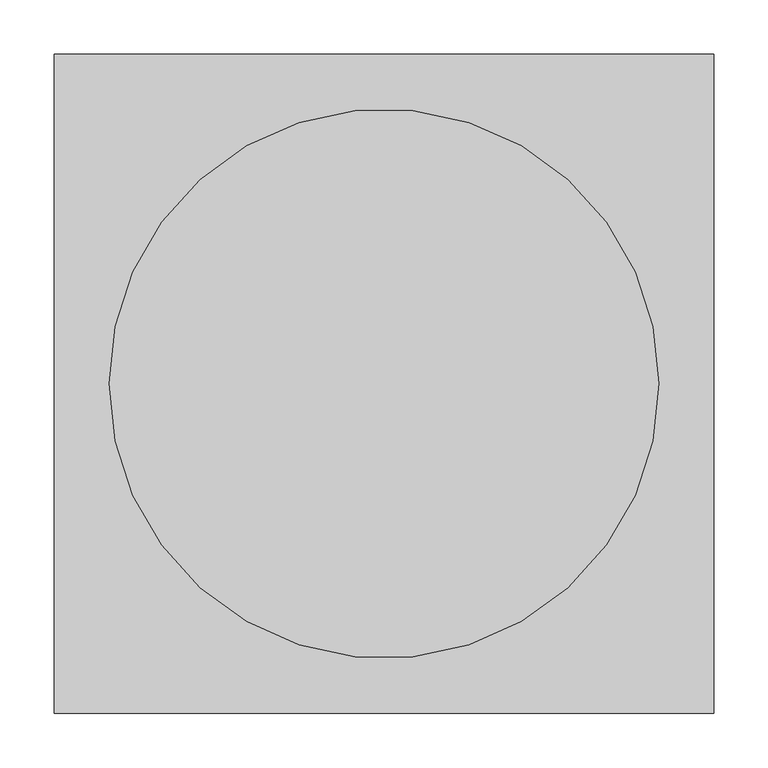
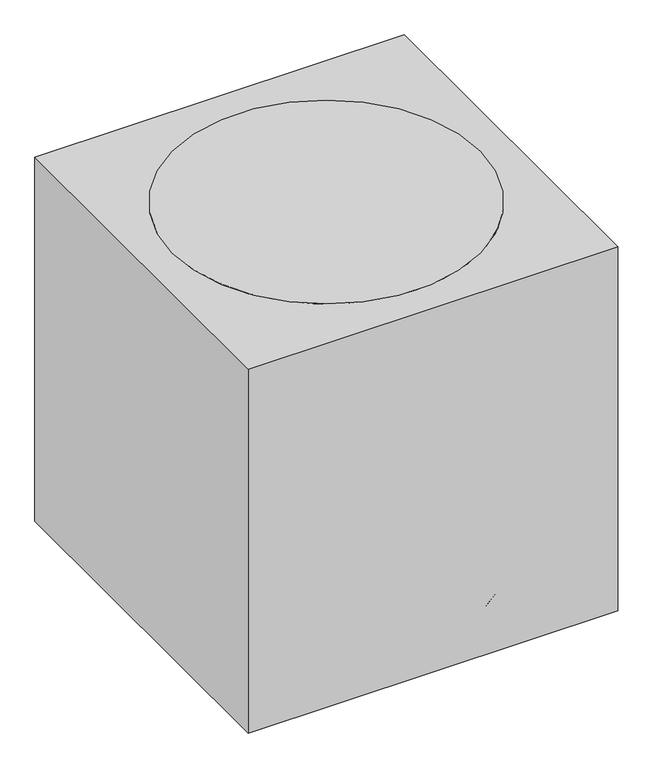
"""IFC4 building model written with IfcOpenShell, lengths in millimetres: proxy geometry, M5030 - Stool, Surgeon, Revolving : M5030 - Stool, Surgeon, Revolving."""

import ifcopenshell
import ifcopenshell.guid

model = None  # the IFC model being written
_history = None  # IfcOwnerHistory: only IFC2X3 demands one
_inside = {}  # id of a spatial element -> (the spatial element, [elements in it])
_under = {}  # id of a project, library or spatial element -> (it, [spatial elements below it])
_declared = {}  # id of a project -> (the project, [libraries it declares])
_typed = {}  # id of a type object -> (the type object, [elements of that type])
_made_of = {}  # id of a material, layer set ... -> (it, [elements and type objects made of it])


def new_model(schema):
    """Start an empty IFC model of exactly this schema.

    Asked for "IFC4X3", IfcOpenShell would pick the latest addendum, in which some entities
    have other attributes; the version numbers below select the first issue.
    IFC2X3 requires an IfcOwnerHistory on every rooted entity: one is made here for all.
    """
    global model, _history
    if schema == "IFC4X3":
        model = ifcopenshell.file(schema_version=(4, 3, 0, 0))
    else:
        model = ifcopenshell.file(schema=schema)
    _inside.clear()
    _under.clear()
    _declared.clear()
    _typed.clear()
    _made_of.clear()
    _history = None
    if model.schema == "IFC2X3":
        org = make("IfcOrganization", Name="unknown")
        user = make(
            "IfcPersonAndOrganization",
            ThePerson=make("IfcPerson", FamilyName="unknown"),
            TheOrganization=org,
        )
        app = make(
            "IfcApplication",
            ApplicationDeveloper=org,
            Version="unknown",
            ApplicationFullName="unknown",
            ApplicationIdentifier="unknown",
        )
        _history = make(
            "IfcOwnerHistory",
            OwningUser=user,
            OwningApplication=app,
            ChangeAction="ADDED",
            CreationDate=0,
        )
    return model


def make(cls, **values):
    """One entity of the class cls with the attributes given. An attribute that is None is left unset."""
    return model.create_entity(
        cls, **{name: value for name, value in values.items() if value is not None}
    )


def rooted(cls, **values):
    """An entity with a GlobalId (a new one), such as an element, a storey or a relation."""
    return make(cls, GlobalId=ifcopenshell.guid.new(), OwnerHistory=_history, **values)


def si_unit(unit_type, name, prefix=None):
    """IfcSIUnit, for example si_unit("LENGTHUNIT", "METRE", prefix="MILLI")."""
    return make("IfcSIUnit", UnitType=unit_type, Prefix=prefix, Name=name)


def assignment(units):
    """IfcUnitAssignment: the units of a project."""
    return None if units is None else make("IfcUnitAssignment", Units=units)


def point(xyz):
    """IfcCartesianPoint."""
    return None if xyz is None else make("IfcCartesianPoint", Coordinates=xyz)


def direction(xyz):
    """IfcDirection."""
    return None if xyz is None else make("IfcDirection", DirectionRatios=xyz)


def frame(location, z_axis=None, x_axis=None):
    """IfcAxis2Placement3D, a coordinate frame: its origin and axes. An axis left out is left unset."""
    return make(
        "IfcAxis2Placement3D",
        Location=point(location),
        Axis=direction(z_axis),
        RefDirection=direction(x_axis),
    )


def frame_2d(location, x_axis=None):
    """IfcAxis2Placement2D, a coordinate frame in the plane: its origin and x axis."""
    return make(
        "IfcAxis2Placement2D", Location=point(location), RefDirection=direction(x_axis)
    )


def origin():
    """The frame at (0, 0, 0) with its axes left unset."""
    return frame((0.0, 0.0, 0.0))


def origin_with_axes():
    """The frame at (0, 0, 0) with the z axis (0, 0, 1) and the x axis (1, 0, 0) written out."""
    return frame((0.0, 0.0, 0.0), z_axis=(0.0, 0.0, 1.0), x_axis=(1.0, 0.0, 0.0))


def origin_2d():
    """The frame at (0, 0) in the plane with its x axis left unset."""
    return frame_2d((0.0, 0.0))


def place(relative_to, where):
    """IfcLocalPlacement: puts the frame where relative to a parent placement (None: the world)."""
    return make(
        "IfcLocalPlacement", PlacementRelTo=relative_to, RelativePlacement=where
    )


def context(
    kind, dimensions, precision=None, world=None, true_north=None, identifier=None
):
    """IfcGeometricRepresentationContext, for example the 3D "Model" context."""
    return make(
        "IfcGeometricRepresentationContext",
        ContextIdentifier=identifier,
        ContextType=kind,
        CoordinateSpaceDimension=dimensions,
        Precision=precision,
        WorldCoordinateSystem=world,
        TrueNorth=true_north,
    )


def project(units=None, contexts=None):
    """IfcProject with its units and contexts."""
    return rooted(
        "IfcProject",
        Name="project",
        RepresentationContexts=contexts,
        UnitsInContext=assignment(units),
    )


def spatial(cls, under=None, at=None, **own):
    """A site, building, storey or space (cls), placed at a placement, below another one or the project."""
    s = rooted(cls, ObjectPlacement=at, **own)
    if under is not None:
        _under.setdefault(under.id(), (under, []))[1].append(s)
    return s


def polyline(points):
    """IfcPolyline through the points."""
    return make("IfcPolyline", Points=[point(p) for p in points])


def circle_curve(where, radius):
    """IfcCircle in the frame where."""
    return make("IfcCircle", Position=where, Radius=radius)


def trimmed(basis, trim1, trim2, sense, master):
    """IfcTrimmedCurve: the piece of a basis curve between two trims."""
    return make(
        "IfcTrimmedCurve",
        BasisCurve=basis,
        Trim1=trim1,
        Trim2=trim2,
        SenseAgreement=sense,
        MasterRepresentation=master,
    )


def segment(curve, same_sense, transition):
    """IfcCompositeCurveSegment."""
    return make(
        "IfcCompositeCurveSegment",
        Transition=transition,
        SameSense=same_sense,
        ParentCurve=curve,
    )


def composite_curve(segments, self_intersect=None):
    """IfcCompositeCurve: segments joined end to end."""
    return make("IfcCompositeCurve", Segments=segments, SelfIntersect=self_intersect)


def outline(outer, holes=None, kind="AREA"):
    """IfcArbitraryClosedProfileDef: a profile drawn as a closed curve; with holes, ...WithVoids."""
    if holes is None:
        return make("IfcArbitraryClosedProfileDef", ProfileType=kind, OuterCurve=outer)
    return make(
        "IfcArbitraryProfileDefWithVoids",
        ProfileType=kind,
        OuterCurve=outer,
        InnerCurves=holes,
    )


def extrude(swept, where, along, depth):
    """IfcExtrudedAreaSolid: the profile swept, set in the frame where, extruded along a direction by depth."""
    return make(
        "IfcExtrudedAreaSolid",
        SweptArea=swept,
        Position=where,
        ExtrudedDirection=direction(along),
        Depth=depth,
    )


def shape(context_of_items, identifier, shape_type, items):
    """IfcShapeRepresentation: the items that make up one representation, for example the "Body"."""
    return make(
        "IfcShapeRepresentation",
        ContextOfItems=context_of_items,
        RepresentationIdentifier=identifier,
        RepresentationType=shape_type,
        Items=items,
    )


def source(mapping_origin, context_of_items, identifier, shape_type, items):
    """IfcRepresentationMap: a shape defined once, which mapped items show again and again."""
    return make(
        "IfcRepresentationMap",
        MappingOrigin=mapping_origin,
        MappedRepresentation=shape(context_of_items, identifier, shape_type, items),
    )


def transform(
    local_origin,
    x_axis=None,
    y_axis=None,
    z_axis=None,
    scale=None,
    scale2=None,
    scale3=None,
    uniform=True,
):
    """IfcCartesianTransformationOperator3D, or its non-uniform kind. x_axis, y_axis, z_axis: its Axis1, 2, 3."""
    if uniform:
        return make(
            "IfcCartesianTransformationOperator3D",
            Axis1=direction(x_axis),
            Axis2=direction(y_axis),
            LocalOrigin=point(local_origin),
            Scale=scale,
            Axis3=direction(z_axis),
        )
    return make(
        "IfcCartesianTransformationOperator3DnonUniform",
        Axis1=direction(x_axis),
        Axis2=direction(y_axis),
        LocalOrigin=point(local_origin),
        Scale=scale,
        Axis3=direction(z_axis),
        Scale2=scale2,
        Scale3=scale3,
    )


def mapped(mapping_source, mapping_target):
    """IfcMappedItem: shows the shape of a source again, moved by a transform."""
    return make(
        "IfcMappedItem", MappingSource=mapping_source, MappingTarget=mapping_target
    )


def made_of(thing, what):
    """Note that an element or type object is made of a material, layer set ...; save() writes the relation."""
    if what is not None:
        _made_of.setdefault(what.id(), (what, []))[1].append(thing)
    return thing


def element(
    cls,
    number,
    at=None,
    inside=None,
    cuts=None,
    type_object=None,
    material=None,
    context=None,
    identifier="Body",
    shape_type=None,
    held_by="IfcProductDefinitionShape",
    body=None,
    shapes=None,
    **own,
):
    """One element of the class cls, such as IfcWall. Its Tag is "e" and its number.

    at: its placement. inside: the storey or other place that contains it. cuts: it is an
    opening in that element (IfcRelVoidsElement). A single representation is given by context,
    identifier, shape_type and body (its items); several are given by shapes. held_by: the class
    of the entity that holds the representations. save() writes the other relations.
    """
    e = rooted(cls, Tag="e%d" % number, ObjectPlacement=at, **own)
    if body is not None:
        shapes = [shape(context, identifier, shape_type, body)]
    if shapes is not None:
        e.Representation = make(held_by, Representations=shapes)
    if inside is not None:
        _inside.setdefault(inside.id(), (inside, []))[1].append(e)
    if cuts is not None:
        rooted(
            "IfcRelVoidsElement", RelatingBuildingElement=cuts, RelatedOpeningElement=e
        )
    if type_object is not None:
        _typed.setdefault(type_object.id(), (type_object, []))[1].append(e)
    return made_of(e, material)


def aggregate(whole, parts):
    """IfcRelAggregates: a whole, such as a stair, and the parts it consists of."""
    return rooted("IfcRelAggregates", RelatingObject=whole, RelatedObjects=parts)


def save(model, path):
    """Write the relations noted so far, then the file.

    IfcRelAggregates (storeys below a building ...), IfcRelContainedInSpatialStructure (elements
    in a storey), IfcRelDefinesByType, IfcRelAssociatesMaterial and IfcRelDeclares: one each for
    every whole, place, type object, material and project.
    """
    for whole, parts in _under.values():
        aggregate(whole, parts)
    for where, things in _inside.values():
        rooted(
            "IfcRelContainedInSpatialStructure",
            RelatedElements=things,
            RelatingStructure=where,
        )
    for kind, things in _typed.values():
        rooted("IfcRelDefinesByType", RelatedObjects=things, RelatingType=kind)
    for what, things in _made_of.values():
        rooted("IfcRelAssociatesMaterial", RelatedObjects=things, RelatingMaterial=what)
    for by, libraries in _declared.values():
        rooted("IfcRelDeclares", RelatingContext=by, RelatedDefinitions=libraries)
    model.write(path)


def specialty_equipment_4e63f546(model_context):
    return source(origin(), model_context, "Body", "SweptSolid", [
        extrude(outline(composite_curve([segment(trimmed(circle_curve(origin_2d(), 254.0), [point((-254.0, 0.0))], [point((254.0, 0.0))], False, "CARTESIAN"), True, "CONTINUOUS"), segment(trimmed(circle_curve(origin_2d(), 254.0), [point((254.0, 0.0))], [point((-254.0, 0.0))], False, "CARTESIAN"), True, "CONTINUOUS")], self_intersect=False)), frame((0.0, 0.0, 584.2), z_axis=(0.0, 0.0, 1.0), x_axis=(1.0, 0.0, 0.0)), (0.0, 0.0, 1.0), 50.8),
        extrude(outline(composite_curve([segment(trimmed(circle_curve(frame_2d((0.0, -25.7612183)), 25.7612183), [point((0.0, -51.5224365))], [point((0.0, 0.0))], False, "CARTESIAN"), True, "CONTINUOUS"), segment(trimmed(circle_curve(frame_2d((0.0, -25.7612183)), 25.7612183), [point((0.0, 0.0))], [point((0.0, -51.5224365))], False, "CARTESIAN"), True, "CONTINUOUS")], self_intersect=False)), frame((203.8559823, 49.544861, 25.7612183), z_axis=(-0.3090169943748919, 0.9510565162951716, 0.0), x_axis=(0.0, 0.0, -1.0)), (0.0, 0.0, 1.0), 31.75),
        extrude(outline(composite_curve([segment(polyline([(-57.1058784, 0.0), (-0.678315, 0.0)]), True, "CONTINUOUS"), segment(trimmed(circle_curve(frame_2d((-28.8920968, 0.0)), 28.2137817), [point((-0.678315, 0.0))], [point((-57.1058784, 0.0))], False, "CARTESIAN"), True, "CONTINUOUS")], self_intersect=False)), frame((256.8155026, 63.4140597, 25.7612183), z_axis=(-0.30901699437489183, 0.9510565162951716, 0.0), x_axis=(0.9510565162951716, 0.30901699437489183, 0.0)), (0.0, 0.0, 1.0), 38.1),
        extrude(outline(composite_curve([segment(trimmed(circle_curve(frame_2d((223.4509477, 72.6028121)), 3.5091751), [point((222.3665529, 75.940236))], [point((224.5353424, 69.2653883))], False, "CARTESIAN"), True, "CONTINUOUS"), segment(trimmed(circle_curve(frame_2d((223.4509477, 72.6028121)), 3.5091751), [point((224.5353424, 69.2653883))], [point((222.3665529, 75.940236))], False, "CARTESIAN"), True, "CONTINUOUS")], self_intersect=False)), frame((0.0, 0.0, 53.975), z_axis=(0.0, 0.0, 1.0), x_axis=(1.0, 0.0, 0.0)), (0.0, 0.0, 1.0), 13.49375),
        extrude(outline(polyline([(230.0293313, 68.0638809), (25.3978935, 1.5750963), (21.4736172, 13.6527769), (226.105055, 80.1415615), (230.0293313, 68.0638809)])), frame((0.0, 0.0, 67.46875), z_axis=(0.0, 0.0, 1.0), x_axis=(1.0, 0.0, 0.0)), (0.0, 0.0, 1.0), 50.8),
        extrude(outline(composite_curve([segment(trimmed(circle_curve(frame_2d((0.0, -25.7612182)), 25.7612183), [point((0.0, -51.5224365))], [point((0.0, 0.0))], False, "CARTESIAN"), True, "CONTINUOUS"), segment(trimmed(circle_curve(frame_2d((0.0, -25.7612182)), 25.7612183), [point((0.0, 0.0))], [point((0.0, -51.5224365))], False, "CARTESIAN"), True, "CONTINUOUS")], self_intersect=False)), frame((110.1149259, -178.5683563, 25.7612183), z_axis=(0.8090169943749846, 0.5877852522924221, 0.0), x_axis=(0.0, 0.0, -1.0)), (0.0, 0.0, 1.0), 31.75),
        extrude(outline(composite_curve([segment(polyline([(-57.1058785, 0.0), (-0.6783149, 0.0)]), True, "CONTINUOUS"), segment(trimmed(circle_curve(frame_2d((-28.8920966, 0.0)), 28.2137817), [point((-0.6783149, 0.0))], [point((-57.1058785, 0.0))], False, "CARTESIAN"), True, "CONTINUOUS")], self_intersect=False)), frame((139.6707094, -224.6500351, 25.7612183), z_axis=(0.8090169943749845, 0.5877852522924222, 0.0), x_axis=(0.5877852522924222, -0.8090169943749845, 0.0)), (0.0, 0.0, 1.0), 38.1),
        extrude(outline(composite_curve([segment(trimmed(circle_curve(frame_2d((138.0995178, -190.0789771)), 3.5091751), [point((140.9385001, -188.0163357))], [point((135.2605355, -192.1416185))], False, "CARTESIAN"), True, "CONTINUOUS"), segment(trimmed(circle_curve(frame_2d((138.0995178, -190.0789771)), 3.5091751), [point((135.2605355, -192.1416185))], [point((140.9385001, -188.0163357))], False, "CARTESIAN"), True, "CONTINUOUS")], self_intersect=False)), frame((0.0, 0.0, 53.975), z_axis=(0.0, 0.0, 1.0), x_axis=(1.0, 0.0, 0.0)), (0.0, 0.0, 1.0), 13.49375),
        extrude(outline(polyline([(135.81557, -197.7379985), (9.3463863, -23.6681006), (19.620275, -16.2036835), (146.0894588, -190.2735815), (135.81557, -197.7379985)])), frame((0.0, 0.0, 67.46875), z_axis=(0.0, 0.0, 1.0), x_axis=(1.0, 0.0, 0.0)), (0.0, 0.0, 1.0), 50.8),
        extrude(outline(composite_curve([segment(trimmed(circle_curve(frame_2d((0.0, -25.7612182)), 25.7612183), [point((0.0, -51.5224365))], [point((0.0, 0.0))], False, "CARTESIAN"), True, "CONTINUOUS"), segment(trimmed(circle_curve(frame_2d((0.0, -25.7612182)), 25.7612183), [point((0.0, 0.0))], [point((0.0, -51.5224365))], False, "CARTESIAN"), True, "CONTINUOUS")], self_intersect=False)), frame((-110.1149259, -178.5683563, 25.7612183), z_axis=(-0.8090169943749151, 0.5877852522925178, 0.0), x_axis=(0.0, 0.0, 1.0)), (0.0, 0.0, 1.0), 31.75),
        extrude(outline(composite_curve([segment(trimmed(circle_curve(frame_2d((28.8920966, 0.0)), 28.2137817), [point((57.1058785, 0.0))], [point((0.6783149, 0.0))], False, "CARTESIAN"), True, "CONTINUOUS"), segment(polyline([(0.6783149, 0.0), (57.1058785, 0.0)]), True, "CONTINUOUS")], self_intersect=False)), frame((-139.6707094, -224.6500351, 25.7612183), z_axis=(-0.809016994374915, 0.5877852522925177, 0.0), x_axis=(0.5877852522925177, 0.809016994374915, 0.0)), (0.0, 0.0, 1.0), 38.1),
        extrude(outline(composite_curve([segment(trimmed(circle_curve(frame_2d((-138.1007518, -190.0780805)), 3.5091751), [point((-135.2617695, -192.1407219))], [point((-140.9397341, -188.0154391))], False, "CARTESIAN"), True, "CONTINUOUS"), segment(trimmed(circle_curve(frame_2d((-138.1007518, -190.0780805)), 3.5091751), [point((-140.9397341, -188.0154391))], [point((-135.2617695, -192.1407219))], False, "CARTESIAN"), True, "CONTINUOUS")], self_intersect=False)), frame((0.0, 0.0, 53.975), z_axis=(0.0, 0.0, 1.0), x_axis=(1.0, 0.0, 0.0)), (0.0, 0.0, 1.0), 13.49375),
        extrude(outline(polyline([(-146.0906928, -190.2726849), (-19.6215091, -16.2027869), (-9.3476203, -23.667204), (-135.8168041, -197.737102), (-146.0906928, -190.2726849)])), frame((0.0, 0.0, 67.46875), z_axis=(0.0, 0.0, 1.0), x_axis=(1.0, 0.0, 0.0)), (0.0, 0.0, 1.0), 50.8),
        extrude(outline(composite_curve([segment(trimmed(circle_curve(frame_2d((0.0, -25.7612183)), 25.7612183), [point((0.0, -51.5224365))], [point((0.0, 0.0))], False, "CARTESIAN"), True, "CONTINUOUS"), segment(trimmed(circle_curve(frame_2d((0.0, -25.7612183)), 25.7612183), [point((0.0, 0.0))], [point((0.0, -51.5224365))], False, "CARTESIAN"), True, "CONTINUOUS")], self_intersect=False)), frame((-203.8559823, 49.544861, 25.7612183), z_axis=(0.3090169943749793, 0.9510565162951433, 0.0), x_axis=(0.0, 0.0, 1.0)), (0.0, 0.0, 1.0), 31.75),
        extrude(outline(composite_curve([segment(trimmed(circle_curve(frame_2d((28.8920968, 0.0)), 28.2137817), [point((57.1058784, 0.0))], [point((0.678315, 0.0))], False, "CARTESIAN"), True, "CONTINUOUS"), segment(polyline([(0.678315, 0.0), (57.1058784, 0.0)]), True, "CONTINUOUS")], self_intersect=False)), frame((-256.8155026, 63.4140597, 25.7612183), z_axis=(0.3090169943749793, 0.9510565162951433, 0.0), x_axis=(0.9510565162951433, -0.3090169943749793, 0.0)), (0.0, 0.0, 1.0), 38.1),
        extrude(outline(composite_curve([segment(trimmed(circle_curve(frame_2d((-223.4504763, 72.6042628)), 3.5091751), [point((-224.5348711, 69.266839))], [point((-222.3660816, 75.9416867))], False, "CARTESIAN"), True, "CONTINUOUS"), segment(trimmed(circle_curve(frame_2d((-223.4504763, 72.6042628)), 3.5091751), [point((-222.3660816, 75.9416867))], [point((-224.5348711, 69.266839))], False, "CARTESIAN"), True, "CONTINUOUS")], self_intersect=False)), frame((0.0, 0.0, 53.975), z_axis=(0.0, 0.0, 1.0), x_axis=(1.0, 0.0, 0.0)), (0.0, 0.0, 1.0), 13.49375),
        extrude(outline(polyline([(-226.1045836, 80.1430121), (-21.4731458, 13.6542275), (-25.3974221, 1.576547), (-230.0288599, 68.0653316), (-226.1045836, 80.1430121)])), frame((0.0, 0.0, 67.46875), z_axis=(0.0, 0.0, 1.0), x_axis=(1.0, 0.0, 0.0)), (0.0, 0.0, 1.0), 50.8),
        extrude(outline(composite_curve([segment(trimmed(circle_curve(frame_2d((234.9499827, 25.7612183)), 25.7612183), [point((260.7112009, 25.7612183))], [point((209.1887644, 25.7612183))], False, "CARTESIAN"), True, "CONTINUOUS"), segment(trimmed(circle_curve(frame_2d((234.9499827, 25.7612183)), 25.7612183), [point((209.1887644, 25.7612183))], [point((260.7112009, 25.7612183))], False, "CARTESIAN"), True, "CONTINUOUS")], self_intersect=False)), frame((-15.875, 0.0, 0.0), z_axis=(1.0, 0.0, 0.0), x_axis=(0.0, 1.0, 0.0)), (0.0, 0.0, 1.0), 31.75),
        extrude(outline(composite_curve([segment(trimmed(circle_curve(frame_2d((234.9499827, 25.7612183)), 28.2137817), [point((206.7362009, 25.7612183))], [point((263.1637644, 25.7612183))], False, "CARTESIAN"), True, "CONTINUOUS"), segment(polyline([(263.1637644, 25.7612183), (206.7362009, 25.7612183)]), True, "CONTINUOUS")], self_intersect=False)), frame((-19.05, 0.0, 0.0), z_axis=(1.0, 0.0, 0.0), x_axis=(0.0, 1.0, 0.0)), (0.0, 0.0, 1.0), 38.1),
        extrude(outline(composite_curve([segment(trimmed(circle_curve(frame_2d((0.0007627, 234.9499827)), 3.5091751), [point((-3.5084124, 234.9499827))], [point((3.5099378, 234.9499827))], False, "CARTESIAN"), True, "CONTINUOUS"), segment(trimmed(circle_curve(frame_2d((0.0007627, 234.9499827)), 3.5091751), [point((3.5099378, 234.9499827))], [point((-3.5084124, 234.9499827))], False, "CARTESIAN"), True, "CONTINUOUS")], self_intersect=False)), frame((0.0, 0.0, 53.975), z_axis=(0.0, 0.0, 1.0), x_axis=(1.0, 0.0, 0.0)), (0.0, 0.0, 1.0), 13.49375),
        extrude(outline(polyline([(6.3503751, 239.8037904), (6.3503751, 24.6415636), (-6.3488498, 24.6415636), (-6.3488498, 239.8037904), (6.3503751, 239.8037904)])), frame((0.0, 0.0, 67.46875), z_axis=(0.0, 0.0, 1.0), x_axis=(1.0, 0.0, 0.0)), (0.0, 0.0, 1.0), 50.8),
        extrude(outline(composite_curve([segment(trimmed(circle_curve(origin_2d(), 25.4466483), [point((-25.4466483, 0.0))], [point((25.4466483, 0.0))], False, "CARTESIAN"), True, "CONTINUOUS"), segment(trimmed(circle_curve(origin_2d(), 25.4466483), [point((25.4466483, 0.0))], [point((-25.4466483, 0.0))], False, "CARTESIAN"), True, "CONTINUOUS")], self_intersect=False)), frame((0.0, 0.0, 67.46875), z_axis=(0.0, 0.0, 1.0), x_axis=(1.0, 0.0, 0.0)), (0.0, 0.0, 1.0), 516.73125),
        extrude(outline(polyline([(304.8, 304.8), (304.8, -304.8), (-304.8, -304.8), (-304.8, 304.8), (304.8, 304.8)])), origin_with_axes(), (0.0, 0.0, 1.0), 635.0),
    ])


if __name__ == "__main__":
    model = new_model("IFC4")
    model_context = context("Model", 3, world=origin())
    ifc_project = project(units=[si_unit("LENGTHUNIT", "METRE", prefix="MILLI")], contexts=[model_context])
    site = spatial("IfcSite", under=ifc_project)
    building = spatial("IfcBuilding", under=site)
    placement = place(None, origin())
    specialty_equipment_shape = specialty_equipment_4e63f546(model_context)
    element("IfcBuildingElementProxy", 1, Name="M5030 - Stool, Surgeon, Revolving : M5030 - Stool, Surgeon, Revolving", ObjectType="M5030 - Stool, Surgeon, Revolving : M5030 - Stool, Surgeon, Revolving", at=placement, inside=building, context=model_context, shape_type="MappedRepresentation", body=[
        mapped(specialty_equipment_shape, transform((0.0, 0.0, 0.0), x_axis=(1.0, 0.0, 0.0), y_axis=(0.0, 1.0, 0.0), z_axis=(0.0, 0.0, 1.0))),
    ])
    save(model, "model.ifc")

# Revit data of these elements
# Type "M5030 - Stool, Surgeon, Revolving : M5030 - Stool, Surgeon, Revolving"
#   Watts2 = "0"
#   Watts1 = "0"
#   Unit_Issue = "EA"
#   UTIL_6_Misc = "-"
#   UTIL_5_NonMedGas = "-"
#   UTIL_4_MiscGas = "-"
#   UTIL_3_MedGas = "-"
#   UTIL_2_Elec = "-"
#   UTIL_1_WaterDrain = "-"
#   Nomenclature = "Stool, Surgeon, Revolving"
#   NSN = "6530"
#   Location [instance default] = ""
#   JSN = "M5030"
#   Fund_Source_VA = "-"
#   Fund_Source_Navy = "-"
#   Fund_Source_Army = "-"
#   Fund_Source_AF = "-"
#   ELEC_Volts2 = "0"
#   ELEC_Volts1 = "0"
#   ELEC_Phase2 = "0"
#   ELEC_Phase1 = "0"
#   ELEC_HertzSwitch = "0"
#   ELEC_HertzDependent = "0"
#   ELEC_Hertz = "0"
#   ELEC_Amps2 = "0"
#   ELEC_Amps1 = "0"
#   DetailDescription = "Revolving stool. Consists of a padded upholstered seat with height adjustment. Unit rotates and is mounted on ball bearing swivel\r\ncasters. Designed for use in examinations, treatment, and surgical procedures."
#   CAT_VA = "C"
#   CAT_Navy = "C"
#   CAT_IHS = "-"
#   CAT_Army = "C"
#   CAT_AF = "C"
#   BTUperhour = "0"
#   Weight_IP = 23
#   DIM_Width_IP = 2' - 0"
#   DIM_Height_IP = 2' - 1"
#   DIM_Depth_IP = 2' - 0"
#   Assembly Code = ""
# Element 1 (IfcBuildingElementProxy, "M5030 - Stool, Surgeon, Revolving : M5030 - Stool, Surgeon, Revolving")
#   Materials on its faces: "Stool metal", "Stool caster", "EquipSpace", "Stool cushion"
# Materials
#   "Stool metal": class "Unassigned", colour RGB 201 201 201, transparency 0, Comments = "Rendering appearance not upgraded "
#   "Stool caster": class "Unassigned", colour RGB 0 0 0, transparency 0, Comments = "Rendering appearance not upgraded "
#   "EquipSpace": class "Unassigned", colour RGB 221 217 195, transparency 0.5
#   "Stool cushion": class "Unassigned", colour RGB 226 128 109, transparency 0, Comments = "Rendering appearance not upgraded "
